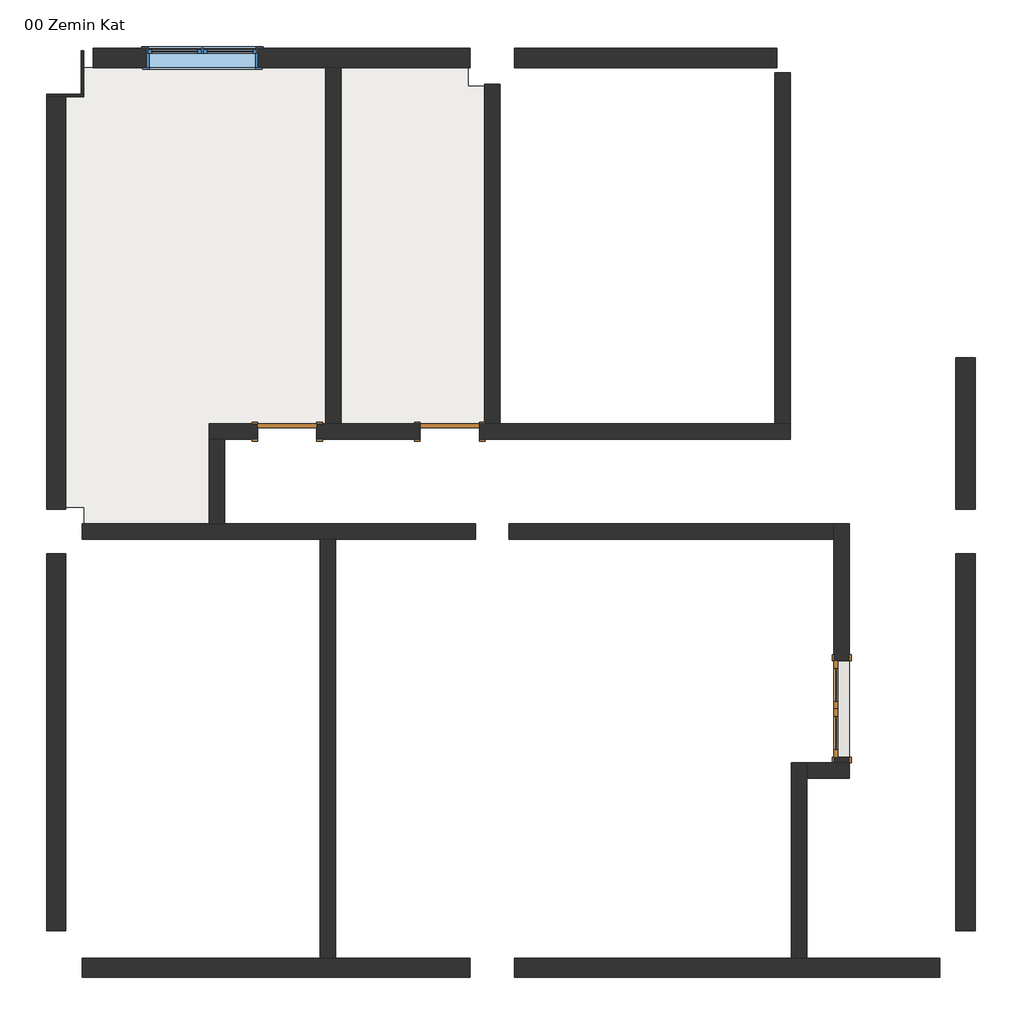
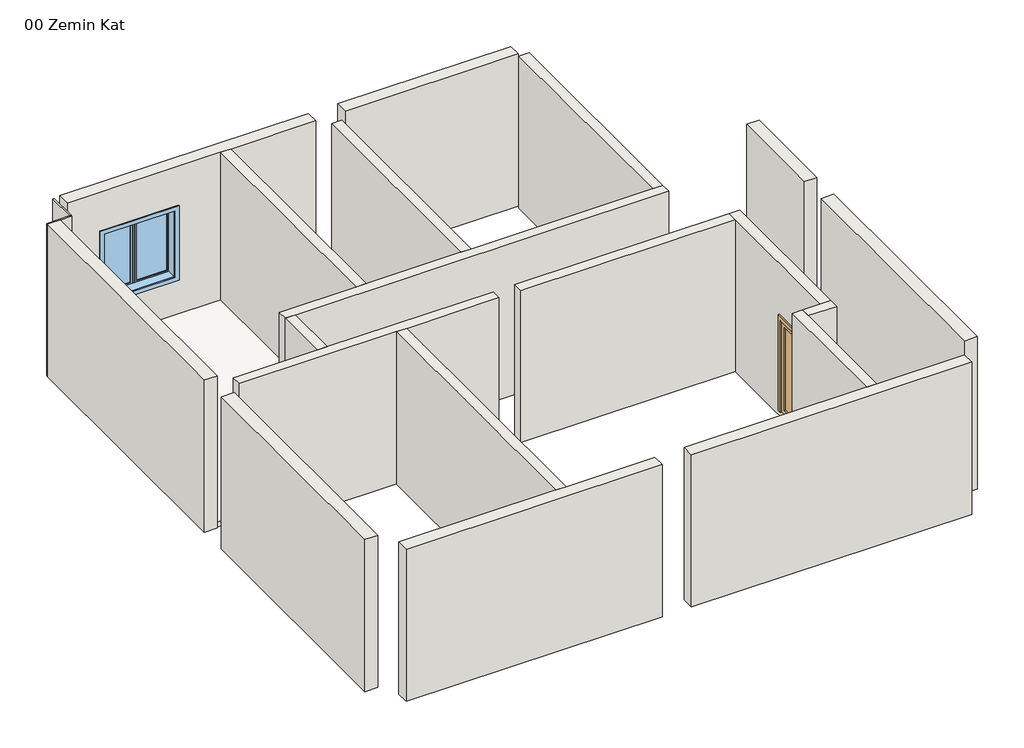
# One storey: 21 walls, 3 doors, 2 slabs, 1 window.
"""IFC4 building model written with IfcOpenShell, lengths in millimetres."""

import ifcopenshell
import ifcopenshell.guid

model = None  # the IFC model being written
_history = None  # IfcOwnerHistory: only IFC2X3 demands one
_inside = {}  # id of a spatial element -> (the spatial element, [elements in it])
_under = {}  # id of a project, library or spatial element -> (it, [spatial elements below it])
_declared = {}  # id of a project -> (the project, [libraries it declares])
_typed = {}  # id of a type object -> (the type object, [elements of that type])
_made_of = {}  # id of a material, layer set ... -> (it, [elements and type objects made of it])


def new_model(schema):
    """Start an empty IFC model of exactly this schema.

    Asked for "IFC4X3", IfcOpenShell would pick the latest addendum, in which some entities
    have other attributes; the version numbers below select the first issue.
    IFC2X3 requires an IfcOwnerHistory on every rooted entity: one is made here for all.
    """
    global model, _history
    if schema == "IFC4X3":
        model = ifcopenshell.file(schema_version=(4, 3, 0, 0))
    else:
        model = ifcopenshell.file(schema=schema)
    _inside.clear()
    _under.clear()
    _declared.clear()
    _typed.clear()
    _made_of.clear()
    _history = None
    if model.schema == "IFC2X3":
        org = make("IfcOrganization", Name="unknown")
        user = make(
            "IfcPersonAndOrganization",
            ThePerson=make("IfcPerson", FamilyName="unknown"),
            TheOrganization=org,
        )
        app = make(
            "IfcApplication",
            ApplicationDeveloper=org,
            Version="unknown",
            ApplicationFullName="unknown",
            ApplicationIdentifier="unknown",
        )
        _history = make(
            "IfcOwnerHistory",
            OwningUser=user,
            OwningApplication=app,
            ChangeAction="ADDED",
            CreationDate=0,
        )
    return model


def make(cls, **values):
    """One entity of the class cls with the attributes given. An attribute that is None is left unset."""
    return model.create_entity(
        cls, **{name: value for name, value in values.items() if value is not None}
    )


def rooted(cls, **values):
    """An entity with a GlobalId (a new one), such as an element, a storey or a relation."""
    return make(cls, GlobalId=ifcopenshell.guid.new(), OwnerHistory=_history, **values)


def si_unit(unit_type, name, prefix=None):
    """IfcSIUnit, for example si_unit("LENGTHUNIT", "METRE", prefix="MILLI")."""
    return make("IfcSIUnit", UnitType=unit_type, Prefix=prefix, Name=name)


def assignment(units):
    """IfcUnitAssignment: the units of a project."""
    return None if units is None else make("IfcUnitAssignment", Units=units)


def point(xyz):
    """IfcCartesianPoint."""
    return None if xyz is None else make("IfcCartesianPoint", Coordinates=xyz)


def direction(xyz):
    """IfcDirection."""
    return None if xyz is None else make("IfcDirection", DirectionRatios=xyz)


def frame(location, z_axis=None, x_axis=None):
    """IfcAxis2Placement3D, a coordinate frame: its origin and axes. An axis left out is left unset."""
    return make(
        "IfcAxis2Placement3D",
        Location=point(location),
        Axis=direction(z_axis),
        RefDirection=direction(x_axis),
    )


def origin():
    """The frame at (0, 0, 0) with its axes left unset."""
    return frame((0.0, 0.0, 0.0))


def origin_with_axes():
    """The frame at (0, 0, 0) with the z axis (0, 0, 1) and the x axis (1, 0, 0) written out."""
    return frame((0.0, 0.0, 0.0), z_axis=(0.0, 0.0, 1.0), x_axis=(1.0, 0.0, 0.0))


def place(relative_to, where):
    """IfcLocalPlacement: puts the frame where relative to a parent placement (None: the world)."""
    return make(
        "IfcLocalPlacement", PlacementRelTo=relative_to, RelativePlacement=where
    )


def context(
    kind, dimensions, precision=None, world=None, true_north=None, identifier=None
):
    """IfcGeometricRepresentationContext, for example the 3D "Model" context."""
    return make(
        "IfcGeometricRepresentationContext",
        ContextIdentifier=identifier,
        ContextType=kind,
        CoordinateSpaceDimension=dimensions,
        Precision=precision,
        WorldCoordinateSystem=world,
        TrueNorth=true_north,
    )


def project(units=None, contexts=None):
    """IfcProject with its units and contexts."""
    return rooted(
        "IfcProject",
        Name="project",
        RepresentationContexts=contexts,
        UnitsInContext=assignment(units),
    )


def spatial(cls, under=None, at=None, **own):
    """A site, building, storey or space (cls), placed at a placement, below another one or the project."""
    s = rooted(cls, ObjectPlacement=at, **own)
    if under is not None:
        _under.setdefault(under.id(), (under, []))[1].append(s)
    return s


def polyline(points):
    """IfcPolyline through the points."""
    return make("IfcPolyline", Points=[point(p) for p in points])


def outline(outer, holes=None, kind="AREA"):
    """IfcArbitraryClosedProfileDef: a profile drawn as a closed curve; with holes, ...WithVoids."""
    if holes is None:
        return make("IfcArbitraryClosedProfileDef", ProfileType=kind, OuterCurve=outer)
    return make(
        "IfcArbitraryProfileDefWithVoids",
        ProfileType=kind,
        OuterCurve=outer,
        InnerCurves=holes,
    )


def extrude(swept, where, along, depth):
    """IfcExtrudedAreaSolid: the profile swept, set in the frame where, extruded along a direction by depth."""
    return make(
        "IfcExtrudedAreaSolid",
        SweptArea=swept,
        Position=where,
        ExtrudedDirection=direction(along),
        Depth=depth,
    )


def faces_of(points, faces, orient=None, outer=None):
    """IfcFace entities. A face is a list of loops; a loop is a list of indices into points, from 0.

    orient and outer hold one flag for each loop. By default every Orientation is true, the
    first loop of a face is its IfcFaceOuterBound and the others are IfcFaceBound.
    """
    made = []
    for i, loops in enumerate(faces):
        bounds = []
        for j, loop in enumerate(loops):
            is_outer = j == 0 if outer is None else outer[i][j]
            bounds.append(
                make(
                    "IfcFaceOuterBound" if is_outer else "IfcFaceBound",
                    Bound=make("IfcPolyLoop", Polygon=[points[k] for k in loop]),
                    Orientation=True if orient is None else orient[i][j],
                )
            )
        made.append(make("IfcFace", Bounds=bounds))
    return made


def faceted_brep(points, faces, orient=None, outer=None, voids=None):
    """IfcFacetedBrep: a solid bounded by flat faces; with voids (closed shells), ...WithVoids."""
    shared = [point(p) for p in points]
    hull = make("IfcClosedShell", CfsFaces=faces_of(shared, faces, orient, outer))
    if voids is None:
        return make("IfcFacetedBrep", Outer=hull)
    return make(
        "IfcFacetedBrepWithVoids",
        Outer=hull,
        Voids=[
            make(cls, CfsFaces=faces_of(shared, fs, o, b)) for cls, fs, o, b in voids
        ],
    )


def shape(context_of_items, identifier, shape_type, items):
    """IfcShapeRepresentation: the items that make up one representation, for example the "Body"."""
    return make(
        "IfcShapeRepresentation",
        ContextOfItems=context_of_items,
        RepresentationIdentifier=identifier,
        RepresentationType=shape_type,
        Items=items,
    )


def source(mapping_origin, context_of_items, identifier, shape_type, items):
    """IfcRepresentationMap: a shape defined once, which mapped items show again and again."""
    return make(
        "IfcRepresentationMap",
        MappingOrigin=mapping_origin,
        MappedRepresentation=shape(context_of_items, identifier, shape_type, items),
    )


def transform(
    local_origin,
    x_axis=None,
    y_axis=None,
    z_axis=None,
    scale=None,
    scale2=None,
    scale3=None,
    uniform=True,
):
    """IfcCartesianTransformationOperator3D, or its non-uniform kind. x_axis, y_axis, z_axis: its Axis1, 2, 3."""
    if uniform:
        return make(
            "IfcCartesianTransformationOperator3D",
            Axis1=direction(x_axis),
            Axis2=direction(y_axis),
            LocalOrigin=point(local_origin),
            Scale=scale,
            Axis3=direction(z_axis),
        )
    return make(
        "IfcCartesianTransformationOperator3DnonUniform",
        Axis1=direction(x_axis),
        Axis2=direction(y_axis),
        LocalOrigin=point(local_origin),
        Scale=scale,
        Axis3=direction(z_axis),
        Scale2=scale2,
        Scale3=scale3,
    )


def mapped(mapping_source, mapping_target):
    """IfcMappedItem: shows the shape of a source again, moved by a transform."""
    return make(
        "IfcMappedItem", MappingSource=mapping_source, MappingTarget=mapping_target
    )


def made_of(thing, what):
    """Note that an element or type object is made of a material, layer set ...; save() writes the relation."""
    if what is not None:
        _made_of.setdefault(what.id(), (what, []))[1].append(thing)
    return thing


def element(
    cls,
    number,
    at=None,
    inside=None,
    cuts=None,
    type_object=None,
    material=None,
    context=None,
    identifier="Body",
    shape_type=None,
    held_by="IfcProductDefinitionShape",
    body=None,
    shapes=None,
    **own,
):
    """One element of the class cls, such as IfcWall. Its Tag is "e" and its number.

    at: its placement. inside: the storey or other place that contains it. cuts: it is an
    opening in that element (IfcRelVoidsElement). A single representation is given by context,
    identifier, shape_type and body (its items); several are given by shapes. held_by: the class
    of the entity that holds the representations. save() writes the other relations.
    """
    e = rooted(cls, Tag="e%d" % number, ObjectPlacement=at, **own)
    if body is not None:
        shapes = [shape(context, identifier, shape_type, body)]
    if shapes is not None:
        e.Representation = make(held_by, Representations=shapes)
    if inside is not None:
        _inside.setdefault(inside.id(), (inside, []))[1].append(e)
    if cuts is not None:
        rooted(
            "IfcRelVoidsElement", RelatingBuildingElement=cuts, RelatedOpeningElement=e
        )
    if type_object is not None:
        _typed.setdefault(type_object.id(), (type_object, []))[1].append(e)
    return made_of(e, material)


def aggregate(whole, parts):
    """IfcRelAggregates: a whole, such as a stair, and the parts it consists of."""
    return rooted("IfcRelAggregates", RelatingObject=whole, RelatedObjects=parts)


def save(model, path):
    """Write the relations noted so far, then the file.

    IfcRelAggregates (storeys below a building ...), IfcRelContainedInSpatialStructure (elements
    in a storey), IfcRelDefinesByType, IfcRelAssociatesMaterial and IfcRelDeclares: one each for
    every whole, place, type object, material and project.
    """
    for whole, parts in _under.values():
        aggregate(whole, parts)
    for where, things in _inside.values():
        rooted(
            "IfcRelContainedInSpatialStructure",
            RelatedElements=things,
            RelatingStructure=where,
        )
    for kind, things in _typed.values():
        rooted("IfcRelDefinesByType", RelatedObjects=things, RelatingType=kind)
    for what, things in _made_of.values():
        rooted("IfcRelAssociatesMaterial", RelatedObjects=things, RelatingMaterial=what)
    for by, libraries in _declared.values():
        rooted("IfcRelDeclares", RelatingContext=by, RelatedDefinitions=libraries)
    model.write(path)


def m_door_double_glass_87eabaac(model_context):
    return source(origin(), model_context, "Body", "SweptSolid", [
        extrude(outline(polyline([(2000.0, -650.0), (0.0, -650.0), (0.0, 0.0), (2000.0, 0.0), (2000.0, -650.0)]), holes=[polyline([(1900.0, -550.0), (1900.0, -100.0), (100.0, -100.0), (100.0, -550.0), (1900.0, -550.0)])]), frame((0.0, 57.38125, 0.0), z_axis=(0.0, 1.0, 0.0), x_axis=(0.0, 0.0, 1.0)), (0.0, 0.0, 1.0), 50.0),
        extrude(outline(polyline([(2000.0, 650.0), (2000.0, 0.0), (0.0, 0.0), (0.0, 650.0), (2000.0, 650.0)]), holes=[polyline([(1900.0, 550.0), (100.0, 550.0), (100.0, 100.0), (1900.0, 100.0), (1900.0, 550.0)])]), frame((0.0, 57.38125, 0.0), z_axis=(0.0, 1.0, 0.0), x_axis=(0.0, 0.0, 1.0)), (0.0, 0.0, 1.0), 50.0),
        extrude(outline(polyline([(100.0, 85.55625), (550.0, 85.55625), (550.0, 79.20625), (100.0, 79.20625), (100.0, 85.55625)])), frame((0.0, 0.0, 100.0), z_axis=(0.0, 0.0, 1.0), x_axis=(1.0, 0.0, 0.0)), (0.0, 0.0, 1.0), 1800.0),
        extrude(outline(polyline([(-550.0, 85.55625), (-100.0, 85.55625), (-100.0, 79.20625), (-550.0, 79.20625), (-550.0, 85.55625)])), frame((0.0, 0.0, 100.0), z_axis=(0.0, 0.0, 1.0), x_axis=(1.0, 0.0, 0.0)), (0.0, 0.0, 1.0), 1800.0),
        extrude(outline(polyline([(0.0, 730.0), (2080.0, 730.0), (2080.0, -730.0), (0.0, -730.0), (0.0, -650.0), (2000.0, -650.0), (2000.0, 650.0), (0.0, 650.0), (0.0, 730.0)])), frame((0.0, 107.38125, 0.0), z_axis=(0.0, 1.0, 0.0), x_axis=(0.0, 0.0, 1.0)), (0.0, 0.0, 1.0), 25.0),
        extrude(outline(polyline([(0.0, 730.0), (2080.0, 730.0), (2080.0, -730.0), (0.0, -730.0), (0.0, -650.0), (2000.0, -650.0), (2000.0, 650.0), (0.0, 650.0), (0.0, 730.0)])), frame((0.0, -127.61875, 0.0), z_axis=(0.0, 1.0, 0.0), x_axis=(0.0, 0.0, 1.0)), (0.0, 0.0, 1.0), 25.0),
    ])


def m_single_flush_43d1bd44(model_context):
    return source(origin(), model_context, "Body", "SweptSolid", [
        extrude(outline(polyline([(2176.0, -476.0), (0.0, -476.0), (0.0, -400.0), (2100.0, -400.0), (2100.0, 400.0), (0.0, 400.0), (0.0, 476.0), (2176.0, 476.0), (2176.0, -476.0)])), frame((0.0, 105.0, 0.0), z_axis=(0.0, 1.0, 0.0), x_axis=(0.0, 0.0, 1.0)), (0.0, 0.0, 1.0), 25.0),
        extrude(outline(polyline([(2176.0, 476.0), (2176.0, -476.0), (0.0, -476.0), (0.0, -400.0), (2100.0, -400.0), (2100.0, 400.0), (0.0, 400.0), (0.0, 476.0), (2176.0, 476.0)])), frame((0.0, -130.0, 0.0), z_axis=(0.0, 1.0, 0.0), x_axis=(0.0, 0.0, 1.0)), (0.0, 0.0, 1.0), 25.0),
        extrude(outline(polyline([(400.0, 54.0), (-400.0, 54.0), (-400.0, 105.0), (400.0, 105.0), (400.0, 54.0)])), origin_with_axes(), (0.0, 0.0, 1.0), 2100.0),
    ])


def m_casement_dbl_with_trim_011da180(model_context):
    return source(origin(), model_context, "Body", "SweptSolid", [
        extrude(outline(polyline([(63.5, 114.175), (686.5, 114.175), (686.5, 101.475), (63.5, 101.475), (63.5, 114.175)])), frame((0.0, 0.0, 978.5), z_axis=(0.0, 0.0, 1.0), x_axis=(1.0, 0.0, 0.0)), (0.0, 0.0, 1.0), 1373.0),
        extrude(outline(polyline([(2395.95, 19.05), (934.05, 19.05), (934.05, 730.95), (2395.95, 730.95), (2395.95, 19.05)]), holes=[polyline([(2351.5, 63.5), (2351.5, 686.5), (978.5, 686.5), (978.5, 63.5), (2351.5, 63.5)])]), frame((0.0, 85.6, 0.0), z_axis=(0.0, 1.0, 0.0), x_axis=(0.0, 0.0, 1.0)), (0.0, 0.0, 1.0), 44.45),
        extrude(outline(polyline([(-819.95, 174.75), (819.95, 174.75), (819.95, 149.05), (-819.95, 149.05), (-819.95, 174.75)])), frame((0.0, 0.0, 915.0), z_axis=(0.0, 0.0, 1.0), x_axis=(1.0, 0.0, 0.0)), (0.0, 0.0, 1.0), 19.05),
        extrude(outline(polyline([(2395.95, -730.95), (2395.95, 730.95), (934.05, 730.95), (934.05, 819.95), (2484.95, 819.95), (2484.95, -819.95), (934.05, -819.95), (934.05, -730.95), (2395.95, -730.95)])), frame((0.0, 149.05, 0.0), z_axis=(0.0, 1.0, 0.0), x_axis=(0.0, 0.0, 1.0)), (0.0, 0.0, 1.0), 13.0),
        extrude(outline(polyline([(2472.25, 807.25), (2472.25, -807.25), (857.75, -807.25), (857.75, 807.25), (2472.25, 807.25)]), holes=[polyline([(2383.25, 718.25), (946.75, 718.25), (946.75, -718.25), (2383.25, -718.25), (2383.25, 718.25)])]), frame((0.0, -129.95, 0.0), z_axis=(0.0, 1.0, 0.0), x_axis=(0.0, 0.0, 1.0)), (0.0, 0.0, 1.0), 19.0),
        extrude(outline(polyline([(-63.5, 101.475), (-686.5, 101.475), (-686.5, 114.175), (-63.5, 114.175), (-63.5, 101.475)])), frame((0.0, 0.0, 978.5), z_axis=(0.0, 0.0, 1.0), x_axis=(1.0, 0.0, 0.0)), (0.0, 0.0, 1.0), 1373.0),
        extrude(outline(polyline([(2395.95, -730.95), (934.05, -730.95), (934.05, -19.05), (2395.95, -19.05), (2395.95, -730.95)]), holes=[polyline([(2351.5, -686.5), (2351.5, -63.5), (978.5, -63.5), (978.5, -686.5), (2351.5, -686.5)])]), frame((0.0, 85.6, 0.0), z_axis=(0.0, 1.0, 0.0), x_axis=(0.0, 0.0, 1.0)), (0.0, 0.0, 1.0), 44.45),
        extrude(outline(polyline([(2415.0, -750.0), (915.0, -750.0), (915.0, 750.0), (2415.0, 750.0), (2415.0, -750.0)]), holes=[polyline([(2383.25, -718.25), (2383.25, 718.25), (946.75, 718.25), (946.75, -718.25), (2383.25, -718.25)])]), frame((0.0, -110.95, 0.0), z_axis=(0.0, 1.0, 0.0), x_axis=(0.0, 0.0, 1.0)), (0.0, 0.0, 1.0), 196.55),
        extrude(outline(polyline([(2415.0, 750.0), (2415.0, -750.0), (915.0, -750.0), (915.0, 750.0), (2415.0, 750.0)]), holes=[polyline([(2395.95, 730.95), (934.05, 730.95), (934.05, -730.95), (2395.95, -730.95), (2395.95, 730.95)])]), frame((0.0, 85.6, 0.0), z_axis=(0.0, 1.0, 0.0), x_axis=(0.0, 0.0, 1.0)), (0.0, 0.0, 1.0), 63.45),
        extrude(outline(polyline([(19.05, 85.6), (-19.05, 85.6), (-19.05, 149.1), (19.05, 149.1), (19.05, 85.6)])), frame((0.0, 0.0, 934.05), z_axis=(0.0, 0.0, 1.0), x_axis=(1.0, 0.0, 0.0)), (0.0, 0.0, 1.0), 1461.9),
    ])


model = new_model("IFC4")

# Units and contexts
model_context = context("Model", 3, world=origin())
ifc_project = project(units=[si_unit("LENGTHUNIT", "METRE", prefix="MILLI")], contexts=[model_context])

# Site, building, storey
site = spatial("IfcSite", under=ifc_project)
building = spatial("IfcBuilding", under=site)
storey = spatial("IfcBuildingStorey", under=building, Name="00 Zemin Kat", Elevation=93780.0)

# Doors
placement = place(None, origin())
m_door_double_glass_shape = m_door_double_glass_87eabaac(model_context)
element("IfcDoor", 1, ObjectType="M_Door-Double-Glass : 130x210cm Kapı", at=placement, inside=storey, context=model_context, shape_type="MappedRepresentation", body=[
    mapped(m_door_double_glass_shape, transform((-4449.1672628, -121.7095574, 93900.0), x_axis=(0.0, 1.0, 0.0), y_axis=(-1.0, 0.0, 0.0), z_axis=(0.0, 0.0, 1.0))),
])
m_single_flush_shape = m_single_flush_43d1bd44(model_context)
element("IfcDoor", 2, ObjectType="M_Single-Flush : 90x210cm Kapı", at=placement, inside=storey, context=model_context, shape_type="MappedRepresentation", body=[
    mapped(m_single_flush_shape, transform((-11954.0485128, 3626.2599093, 93780.0), x_axis=(1.0, 0.0, 0.0), y_axis=(0.0, 1.0, 0.0), z_axis=(0.0, 0.0, 1.0))),
])
element("IfcDoor", 3, ObjectType="M_Single-Flush : 90x210cm Kapı", at=placement, inside=storey, context=model_context, shape_type="MappedRepresentation", body=[
    mapped(m_single_flush_shape, transform((-9754.0485128, 3626.2599093, 93780.0), x_axis=(1.0, 0.0, 0.0), y_axis=(0.0, 1.0, 0.0), z_axis=(0.0, 0.0, 1.0))),
])

# Slabs
element("IfcSlab", 4, ObjectType="10cm Parke", at=placement, inside=storey, context=model_context, shape_type="SweptSolid", body=[
    extrude(outline(polyline([(-14699.0485128, 8548.2904426), (-11434.0485128, 8548.2904426), (-11434.0485128, 3731.2599093), (-13009.0485128, 3731.2599093), (-13009.0485128, 2383.2904426), (-14699.0485128, 2383.2904426), (-14699.0485128, 2608.2904426), (-14949.0485128, 2608.2904426), (-14949.0485128, 8148.2904426), (-14699.0485128, 8148.2904426), (-14699.0485128, 8548.2904426)])), frame((0.0, 0.0, 93780.0), z_axis=(0.0, 0.0, 1.0), x_axis=(1.0, 0.0, 0.0)), (0.0, 0.0, 1.0), 100.0),
])
element("IfcSlab", 5, ObjectType="10cm Seramik", at=placement, inside=storey, context=model_context, shape_type="SweptSolid", body=[
    extrude(outline(polyline([(-9509.0485128, 8548.2904426), (-9509.0485128, 8298.2904426), (-9284.0485128, 8298.2904426), (-9284.0485128, 3731.2599093), (-11224.0485128, 3731.2599093), (-11224.0485128, 8548.2904426), (-9509.0485128, 8548.2904426)])), frame((0.0, 0.0, 93780.0), z_axis=(0.0, 0.0, 1.0), x_axis=(1.0, 0.0, 0.0)), (0.0, 0.0, 1.0), 100.0),
])

# Walls
element("IfcWall", 6, ObjectType="Dış Duvar_26cm", at=placement, inside=storey, context=model_context, shape_type="Brep", body=[
    faceted_brep([(-14579.0485128, 8548.2904426, 93780.0), (-11434.0485128, 8548.2904426, 93780.0), (-11224.0485128, 8548.2904426, 93780.0), (-9479.0485128, 8548.2904426, 93780.0), (-9479.0485128, 8548.2904426, 97080.0), (-11224.0485128, 8548.2904426, 97080.0), (-11434.0485128, 8548.2904426, 97080.0), (-14579.0485128, 8548.2904426, 97080.0), (-12351.5235128, 8548.2904426, 96180.0), (-12351.5235128, 8548.2904426, 94680.0), (-13851.5235128, 8548.2904426, 94680.0), (-13851.5235128, 8548.2904426, 96180.0), (-14579.0485128, 8808.2904426, 93780.0), (-14579.0485128, 8808.2904426, 97080.0), (-9479.0485128, 8808.2904426, 97080.0), (-9479.0485128, 8808.2904426, 93780.0), (-12351.5235128, 8808.2904426, 96180.0), (-13851.5235128, 8808.2904426, 96180.0), (-13851.5235128, 8808.2904426, 94680.0), (-12351.5235128, 8808.2904426, 94680.0)], [[[0, 1, 2, 3, 4, 5, 6, 7], [8, 9, 10, 11]], [[12, 13, 14, 15], [16, 17, 18, 19]], [[3, 2, 1, 0, 12, 15]], [[4, 3, 15, 14]], [[7, 6, 5, 4, 14, 13]], [[0, 7, 13, 12]], [[9, 8, 16, 19]], [[10, 9, 19, 18]], [[11, 10, 18, 17]], [[8, 11, 17, 16]]]),
])
element("IfcWall", 7, ObjectType="Dış Duvar_26cm", at=placement, inside=storey, context=model_context, shape_type="SweptSolid", body=[
    extrude(outline(polyline([(-5329.0485128, 8548.2904426), (-8879.0485128, 8548.2904426), (-8879.0485128, 8808.2904426), (-5329.0485128, 8808.2904426), (-5329.0485128, 8548.2904426)])), frame((0.0, 0.0, 93780.0), z_axis=(0.0, 0.0, 1.0), x_axis=(1.0, 0.0, 0.0)), (0.0, 0.0, 1.0), 3300.0),
])
element("IfcWall", 8, ObjectType="Dış Duvar_26cm", at=placement, inside=storey, context=model_context, shape_type="SweptSolid", body=[
    extrude(outline(polyline([(-2909.0485128, 2578.2904426), (-2909.0485128, 4628.2904426), (-2649.0485128, 4628.2904426), (-2649.0485128, 2578.2904426), (-2909.0485128, 2578.2904426)])), frame((0.0, 0.0, 93780.0), z_axis=(0.0, 0.0, 1.0), x_axis=(1.0, 0.0, 0.0)), (0.0, 0.0, 1.0), 3300.0),
])
element("IfcWall", 9, ObjectType="Dış Duvar_26cm", at=placement, inside=storey, context=model_context, shape_type="SweptSolid", body=[
    extrude(outline(polyline([(-2909.0485128, -3121.7095574), (-2909.0485128, 1978.2904426), (-2649.0485128, 1978.2904426), (-2649.0485128, -3121.7095574), (-2909.0485128, -3121.7095574)])), frame((0.0, 0.0, 93780.0), z_axis=(0.0, 0.0, 1.0), x_axis=(1.0, 0.0, 0.0)), (0.0, 0.0, 1.0), 3300.0),
])
element("IfcWall", 10, ObjectType="Dış Duvar_26cm", at=placement, inside=storey, context=model_context, shape_type="Brep", body=[
    faceted_brep([(-3129.0485128, -3491.7095574, 93780.0), (-4926.5485128, -3491.7095574, 93780.0), (-5136.5485128, -3491.7095574, 93780.0), (-8879.0485128, -3491.7095574, 93780.0), (-8879.0485128, -3491.7095574, 97080.0), (-5136.5485128, -3491.7095574, 97080.0), (-4926.5485128, -3491.7095574, 97080.0), (-3129.0485128, -3491.7095574, 97080.0), (-3129.0485128, -3751.7095574, 93780.0), (-3129.0485128, -3751.7095574, 97080.0), (-8879.0485128, -3751.7095574, 97080.0), (-8879.0485128, -3751.7095574, 93780.0)], [[[0, 1, 2, 3, 4, 5, 6, 7]], [[8, 9, 10, 11]], [[3, 2, 1, 0, 8, 11]], [[4, 3, 11, 10]], [[7, 6, 5, 4, 10, 9]], [[0, 7, 9, 8]]]),
])
element("IfcWall", 11, ObjectType="Dış Duvar_26cm", at=placement, inside=storey, context=model_context, shape_type="Brep", body=[
    faceted_brep([(-9479.0485128, -3491.7095574, 93780.0), (-11299.0485128, -3491.7095574, 93780.0), (-11509.0485128, -3491.7095574, 93780.0), (-14729.0485128, -3491.7095574, 93780.0), (-14729.0485128, -3491.7095574, 97080.0), (-11509.0485128, -3491.7095574, 97080.0), (-11299.0485128, -3491.7095574, 97080.0), (-9479.0485128, -3491.7095574, 97080.0), (-9479.0485128, -3751.7095574, 93780.0), (-9479.0485128, -3751.7095574, 97080.0), (-14729.0485128, -3751.7095574, 97080.0), (-14729.0485128, -3751.7095574, 93780.0)], [[[0, 1, 2, 3, 4, 5, 6, 7]], [[8, 9, 10, 11]], [[3, 2, 1, 0, 8, 11]], [[4, 3, 11, 10]], [[7, 6, 5, 4, 10, 9]], [[0, 7, 9, 8]]]),
])
element("IfcWall", 12, ObjectType="Dış Duvar_26cm", at=placement, inside=storey, context=model_context, shape_type="SweptSolid", body=[
    extrude(outline(polyline([(-14949.0485128, 1978.2904426), (-14949.0485128, -3121.7095574), (-15209.0485128, -3121.7095574), (-15209.0485128, 1978.2904426), (-14949.0485128, 1978.2904426)])), frame((0.0, 0.0, 93780.0), z_axis=(0.0, 0.0, 1.0), x_axis=(1.0, 0.0, 0.0)), (0.0, 0.0, 1.0), 3300.0),
])
element("IfcWall", 13, ObjectType="Dış Duvar_26cm", at=placement, inside=storey, context=model_context, shape_type="SweptSolid", body=[
    extrude(outline(polyline([(-14949.0485128, 8155.7904426), (-14949.0485128, 2578.2904426), (-15209.0485128, 2578.2904426), (-15209.0485128, 8155.7904426), (-14949.0485128, 8155.7904426)])), frame((0.0, 0.0, 93780.0), z_axis=(0.0, 0.0, 1.0), x_axis=(1.0, 0.0, 0.0)), (0.0, 0.0, 1.0), 3300.0),
])
element("IfcWall", 14, ObjectType="İç Duvar_21cm", at=placement, inside=storey, context=model_context, shape_type="SweptSolid", body=[
    extrude(outline(polyline([(-11434.0485128, 3731.2599093), (-11434.0485128, 8548.2904426), (-11224.0485128, 8548.2904426), (-11224.0485128, 3731.2599093), (-11434.0485128, 3731.2599093)])), frame((0.0, 0.0, 93780.0), z_axis=(0.0, 0.0, 1.0), x_axis=(1.0, 0.0, 0.0)), (0.0, 0.0, 1.0), 3300.0),
])
element("IfcWall", 15, ObjectType="İç Duvar_21cm", at=placement, inside=storey, context=model_context, shape_type="Brep", body=[
    faceted_brep([(-9354.0485128, 3521.2599093, 95880.0), (-9354.0485128, 3521.2599093, 93780.0), (-5144.0485128, 3521.2599093, 93780.0), (-5144.0485128, 3521.2599093, 97080.0), (-12799.0485128, 3521.2599093, 97080.0), (-13009.0485128, 3521.2599093, 97080.0), (-13009.0485128, 3521.2599093, 93780.0), (-12799.0485128, 3521.2599093, 93780.0), (-12354.0485128, 3521.2599093, 93780.0), (-12354.0485128, 3521.2599093, 95880.0), (-11554.0485128, 3521.2599093, 95880.0), (-11554.0485128, 3521.2599093, 93780.0), (-10154.0485128, 3521.2599093, 93780.0), (-10154.0485128, 3521.2599093, 95880.0), (-5144.0485128, 3731.2599093, 93780.0), (-5354.0485128, 3731.2599093, 93780.0), (-9074.0485128, 3731.2599093, 93780.0), (-9284.0485128, 3731.2599093, 93780.0), (-9354.0485128, 3731.2599093, 93780.0), (-9354.0485128, 3731.2599093, 95880.0), (-10154.0485128, 3731.2599093, 95880.0), (-10154.0485128, 3731.2599093, 93780.0), (-11224.0485128, 3731.2599093, 93780.0), (-11434.0485128, 3731.2599093, 93780.0), (-11554.0485128, 3731.2599093, 93780.0), (-11554.0485128, 3731.2599093, 95880.0), (-12354.0485128, 3731.2599093, 95880.0), (-12354.0485128, 3731.2599093, 93780.0), (-13009.0485128, 3731.2599093, 93780.0), (-13009.0485128, 3731.2599093, 97080.0), (-11434.0485128, 3731.2599093, 97080.0), (-11224.0485128, 3731.2599093, 97080.0), (-9284.0485128, 3731.2599093, 97080.0), (-9074.0485128, 3731.2599093, 97080.0), (-5354.0485128, 3731.2599093, 97080.0), (-5144.0485128, 3731.2599093, 97080.0)], [[[0, 1, 2, 3, 4, 5, 6, 7, 8, 9, 10, 11, 12, 13]], [[14, 15, 16, 17, 18, 19, 20, 21, 22, 23, 24, 25, 26, 27, 28, 29, 30, 31, 32, 33, 34, 35]], [[8, 7, 6, 28, 27]], [[12, 11, 24, 23, 22, 21]], [[2, 1, 18, 17, 16, 15, 14]], [[5, 4, 3, 35, 34, 33, 32, 31, 30, 29]], [[3, 2, 14, 35]], [[6, 5, 29, 28]], [[25, 24, 11, 10]], [[26, 25, 10, 9]], [[27, 26, 9, 8]], [[19, 18, 1, 0]], [[20, 19, 0, 13]], [[21, 20, 13, 12]]]),
])
element("IfcWall", 16, ObjectType="İç Duvar_21cm", at=placement, inside=storey, context=model_context, shape_type="SweptSolid", body=[
    extrude(outline(polyline([(-5144.0485128, 8478.2904426), (-5144.0485128, 3731.2599093), (-5354.0485128, 3731.2599093), (-5354.0485128, 8478.2904426), (-5144.0485128, 8478.2904426)])), frame((0.0, 0.0, 93780.0), z_axis=(0.0, 0.0, 1.0), x_axis=(1.0, 0.0, 0.0)), (0.0, 0.0, 1.0), 3300.0),
])
element("IfcWall", 17, ObjectType="İç Duvar_21cm", at=placement, inside=storey, context=model_context, shape_type="SweptSolid", body=[
    extrude(outline(polyline([(-9284.0485128, 3731.2599093), (-9284.0485128, 8327.5055023), (-9074.0485128, 8327.5055023), (-9074.0485128, 3731.2599093), (-9284.0485128, 3731.2599093)])), frame((0.0, 0.0, 93780.0), z_axis=(0.0, 0.0, 1.0), x_axis=(1.0, 0.0, 0.0)), (0.0, 0.0, 1.0), 3300.0),
])
element("IfcWall", 18, ObjectType="İç Duvar_21cm", at=placement, inside=storey, context=model_context, shape_type="SweptSolid", body=[
    extrude(outline(polyline([(-13009.0485128, 2383.2904426), (-13009.0485128, 3521.2599093), (-12799.0485128, 3521.2599093), (-12799.0485128, 2383.2904426), (-13009.0485128, 2383.2904426)])), frame((0.0, 0.0, 93780.0), z_axis=(0.0, 0.0, 1.0), x_axis=(1.0, 0.0, 0.0)), (0.0, 0.0, 1.0), 3300.0),
])
element("IfcWall", 19, ObjectType="İç Duvar_21cm", at=placement, inside=storey, context=model_context, shape_type="Brep", body=[
    faceted_brep([(-9404.0485128, 2383.2904426, 93780.0), (-12799.0485128, 2383.2904426, 93780.0), (-13009.0485128, 2383.2904426, 93780.0), (-14729.0485128, 2383.2904426, 93780.0), (-14729.0485128, 2383.2904426, 97080.0), (-13009.0485128, 2383.2904426, 97080.0), (-12799.0485128, 2383.2904426, 97080.0), (-9404.0485128, 2383.2904426, 97080.0), (-9404.0485128, 2173.2904426, 93780.0), (-9404.0485128, 2173.2904426, 97080.0), (-11299.0485128, 2173.2904426, 97080.0), (-11509.0485128, 2173.2904426, 97080.0), (-14729.0485128, 2173.2904426, 97080.0), (-14729.0485128, 2173.2904426, 93780.0), (-11509.0485128, 2173.2904426, 93780.0), (-11299.0485128, 2173.2904426, 93780.0)], [[[0, 1, 2, 3, 4, 5, 6, 7]], [[8, 9, 10, 11, 12, 13, 14, 15]], [[3, 2, 1, 0, 8, 15, 14, 13]], [[4, 3, 13, 12]], [[7, 6, 5, 4, 12, 11, 10, 9]], [[0, 7, 9, 8]]]),
])
element("IfcWall", 20, ObjectType="İç Duvar_21cm", at=placement, inside=storey, context=model_context, shape_type="SweptSolid", body=[
    extrude(outline(polyline([(-11509.0485128, -3491.7095574), (-11509.0485128, 2173.2904426), (-11299.0485128, 2173.2904426), (-11299.0485128, -3491.7095574), (-11509.0485128, -3491.7095574)])), frame((0.0, 0.0, 93780.0), z_axis=(0.0, 0.0, 1.0), x_axis=(1.0, 0.0, 0.0)), (0.0, 0.0, 1.0), 3300.0),
])
element("IfcWall", 21, ObjectType="İç Duvar_21cm", at=placement, inside=storey, context=model_context, shape_type="Brep", body=[
    faceted_brep([(-4926.5485128, -3491.7095574, 93780.0), (-4926.5485128, -1056.7095574, 93780.0), (-4926.5485128, -846.7095574, 93780.0), (-4926.5485128, -846.7095574, 97080.0), (-4926.5485128, -1056.7095574, 97080.0), (-4926.5485128, -3491.7095574, 97080.0), (-5136.5485128, -3491.7095574, 93780.0), (-5136.5485128, -3491.7095574, 97080.0), (-5136.5485128, -846.7095574, 97080.0), (-5136.5485128, -846.7095574, 93780.0)], [[[0, 1, 2, 3, 4, 5]], [[6, 7, 8, 9]], [[2, 1, 0, 6, 9]], [[5, 4, 3, 8, 7]], [[0, 5, 7, 6]], [[3, 2, 9, 8]]]),
])
element("IfcWall", 22, ObjectType="İç Duvar_21cm", at=placement, inside=storey, context=model_context, shape_type="Brep", body=[
    faceted_brep([(-4926.5485128, -1056.7095574, 93780.0), (-4346.5485128, -1056.7095574, 93780.0), (-4346.5485128, -1056.7095574, 97080.0), (-4926.5485128, -1056.7095574, 97080.0), (-4926.5485128, -846.7095574, 93780.0), (-4926.5485128, -846.7095574, 97080.0), (-4556.5485128, -846.7095574, 97080.0), (-4346.5485128, -846.7095574, 97080.0), (-4346.5485128, -846.7095574, 93780.0), (-4556.5485128, -846.7095574, 93780.0)], [[[0, 1, 2, 3]], [[4, 5, 6, 7, 8, 9]], [[1, 0, 4, 9, 8]], [[3, 2, 7, 6, 5]], [[0, 3, 5, 4]], [[2, 1, 8, 7]]]),
])
element("IfcWall", 23, ObjectType="İç Duvar_21cm", at=placement, inside=storey, context=model_context, shape_type="Brep", body=[
    faceted_brep([(-4346.5485128, -846.7095574, 93780.0), (-4346.5485128, 2383.2904426, 93780.0), (-4346.5485128, 2383.2904426, 97080.0), (-4346.5485128, -846.7095574, 97080.0), (-4346.5485128, 528.2904426, 93900.0), (-4346.5485128, -771.7095574, 93900.0), (-4346.5485128, -771.7095574, 95900.0), (-4346.5485128, 528.2904426, 95900.0), (-4556.5485128, 2383.2904426, 93780.0), (-4556.5485128, 2173.2904426, 93780.0), (-4556.5485128, -846.7095574, 93780.0), (-4556.5485128, -846.7095574, 97080.0), (-4556.5485128, 2173.2904426, 97080.0), (-4556.5485128, 2383.2904426, 97080.0), (-4556.5485128, -771.7095574, 93900.0), (-4556.5485128, 528.2904426, 93900.0), (-4556.5485128, 528.2904426, 95900.0), (-4556.5485128, -771.7095574, 95900.0)], [[[0, 1, 2, 3], [4, 5, 6, 7]], [[8, 9, 10, 11, 12, 13], [14, 15, 16, 17]], [[1, 0, 10, 9, 8]], [[3, 2, 13, 12, 11]], [[0, 3, 11, 10]], [[2, 1, 8, 13]], [[14, 5, 4, 15]], [[15, 4, 7, 16]], [[16, 7, 6, 17]], [[5, 14, 17, 6]]]),
])
element("IfcWall", 24, ObjectType="İç Duvar_21cm", at=placement, inside=storey, context=model_context, shape_type="SweptSolid", body=[
    extrude(outline(polyline([(-8954.0485128, 2383.2904426), (-4556.5485128, 2383.2904426), (-4556.5485128, 2173.2904426), (-8954.0485128, 2173.2904426), (-8954.0485128, 2383.2904426)])), frame((0.0, 0.0, 93780.0), z_axis=(0.0, 0.0, 1.0), x_axis=(1.0, 0.0, 0.0)), (0.0, 0.0, 1.0), 3300.0),
])
element("IfcWall", 25, ObjectType="Kolon Çevresi 3cm", at=placement, inside=storey, context=model_context, shape_type="Brep", body=[
    faceted_brep([(-15209.0485128, 8155.7904426, 93780.0), (-14949.0485128, 8155.7904426, 93780.0), (-14706.5485128, 8155.7904426, 93780.0), (-14706.5485128, 8155.7904426, 97080.0), (-14949.0485128, 8155.7904426, 97080.0), (-15209.0485128, 8155.7904426, 97080.0), (-15209.0485128, 8185.7904426, 93780.0), (-15209.0485128, 8185.7904426, 97080.0), (-14736.5485128, 8185.7904426, 97080.0), (-14706.5485128, 8185.7904426, 97080.0), (-14706.5485128, 8185.7904426, 93780.0), (-14736.5485128, 8185.7904426, 93780.0)], [[[0, 1, 2, 3, 4, 5]], [[6, 7, 8, 9, 10, 11]], [[2, 1, 0, 6, 11, 10]], [[5, 4, 3, 9, 8, 7]], [[0, 5, 7, 6]], [[3, 2, 10, 9]]]),
])
element("IfcWall", 26, ObjectType="Kolon Çevresi 3cm", at=placement, inside=storey, context=model_context, shape_type="SweptSolid", body=[
    extrude(outline(polyline([(-14706.5485128, 8778.2904426), (-14706.5485128, 8185.7904426), (-14736.5485128, 8185.7904426), (-14736.5485128, 8778.2904426), (-14706.5485128, 8778.2904426)])), frame((0.0, 0.0, 93780.0), z_axis=(0.0, 0.0, 1.0), x_axis=(1.0, 0.0, 0.0)), (0.0, 0.0, 1.0), 3300.0),
])

# Window
m_casement_dbl_with_trim_shape = m_casement_dbl_with_trim_011da180(model_context)
element("IfcWindow", 27, ObjectType="M_Casement Dbl with Trim : 150x150cm Pencere", at=placement, inside=storey, context=model_context, shape_type="MappedRepresentation", body=[
    mapped(m_casement_dbl_with_trim_shape, transform((-13101.5235128, 8659.2404426, 93765.0), x_axis=(1.0, 0.0, 0.0), y_axis=(0.0, 1.0, 0.0), z_axis=(0.0, 0.0, 1.0))),
])

save(model, "model.ifc")

# Revit data of these elements
# Project information
#   Project Issue Date = "Issue Date"
#   Project Status = "Project Status"
#   Client Name = "Owner"
#   Project Address = "Enter address here"
#   Project Name = "Project Name"
#   Project Number = "0001"
# Type "M_Door-Double-Glass : 130x210cm Kapı"
#   Type Mark = "42"
#   Construction Type Id = "opn-d45"
#   Assembly Code = "C1020"
#   Analytic Construction = "Wood frame, double glass door "
#   W = 65.00 cm
#   Thickness = 5.00 cm
#   Thermal Resistance (R) = 0.31964 (m²·K)/W
#   Swing Angle [instance default] = 90.00°
#   Heat Transfer Coefficient (U) = 3.12872 W/(m²·K)
#   Height = 200.00 cm
#   Bottom Rail = 10.00 cm
#   Top Rail = 10.00 cm
#   Stiles = 10.00 cm
#   Trim Projection = 2.50 cm
#   Trim Width = 8.00 cm
#   Width = 130.00 cm
#   Define Thermal Properties by = 1
#   Glazing = Glass
#   Panel Material = Wood - Birch - Solid Stained Light Low Gloss
#   Trim Material = Paint - Sienna
#   Visual Light Transmittance = 0
#   Solar Heat Gain Coefficient = 0
#   Function = (empty or 0)
#   Wall Closure = (empty or 0)
# Type "M_Single-Flush : 90x210cm Kapı"
#   Type Mark = "40"
#   Construction Type Id = "MDOOR"
#   Analytic Construction = "Metal"
#   Thickness = 5.10 cm
#   Heat Transfer Coefficient (U) = 3.7021 W/(m²·K)
#   Height = 210.00 cm
#   Trim Projection Ext = 2.50 cm
#   Trim Projection Int = 2.50 cm
#   Trim Width = 7.60 cm
#   Width = 80.00 cm
#   Define Thermal Properties by = 1
#   Door Material = Door - Panel
#   Frame Material = Door - Frame
#   Visual Light Transmittance = 0
#   Solar Heat Gain Coefficient = 0
#   Function = (empty or 0)
#   Wall Closure = (empty or 0)
# Type "10cm Parke"
#   Function = 0
#   Layers, outside or top first: 2.00 cm "PARKE" (function 5); 8.00 cm "ŞAP" (function 4)
# Type "10cm Seramik"
#   Function = 0
#   Layers, outside or top first: 2.00 cm "SERAMİK" (function 5); 8.00 cm "ŞAP" (function 4)
# Type "Dış Duvar_26cm"
#   Layers, outside or top first: 1.50 cm "BOYA" (function 5); 1.50 cm "SIVA" (function 4); 20.00 cm "Brick, Common" (function 1); 1.50 cm "SIVA" (function 4); 1.50 cm "BOYA" (function 5)
# Type "İç Duvar_21cm"
#   Layers, outside or top first: 1.50 cm "BOYA" (function 5); 1.50 cm "SIVA" (function 4); 15.00 cm "Brick, Common" (function 1); 1.50 cm "SIVA" (function 4); 1.50 cm "BOYA" (function 5)
# Type "Kolon Çevresi 3cm"
#   Layers, outside or top first: 1.50 cm "BOYA" (function 5); 1.50 cm "SIVA" (function 4)
# Type "M_Casement Dbl with Trim : 150x150cm Pencere"
#   Type Mark = "20"
#   Construction Type Id = "GSP4R"
#   Analytic Construction = "1/8 in Pilkington single glazing"
#   Visual Light Transmittance = 0.9
#   Solar Heat Gain Coefficient = 0.78
#   Heat Transfer Coefficient (U) = 3.6886 W/(m²·K)
#   Height = 150.00 cm
#   Default Sill Height = 91.50 cm
#   Trim Projection - Ext. = 1.30 cm
#   Trim Projection - Int. = 1.90 cm
#   Trim Width - Exterior = 8.90 cm
#   Trim Width - Interior = 8.90 cm
#   Width = 150.00 cm
#   Window Inset = 1.90 cm
#   Define Thermal Properties by = 1
#   Glass Pane Material = Glass
#   Sash = Sash
#   Trim Exterior Material = Trim
#   Trim Interior Material = Trim
#   Wall Closure = (empty or 0)
# Element 1 (IfcDoor, "M_Door-Double-Glass : 130x210cm Kapı")
#   Swing Angle = 90.00°
#   Phase Created = New Construction
#   Materials on its faces: "Wood - Birch - Solid Stained Light Low Gloss", "Paint - Sienna", "Glass"
# Elements 2, 3 (IfcDoor, "M_Single-Flush : 90x210cm Kapı")
#   Phase Created = New Construction
#   Materials on its faces: "Door - Frame", "Door - Panel"
# Element 4 (IfcSlab, "10cm Parke")
#   built-in parameter 1001955 = 1.5708 (stored number, unit not read)
#   Height Offset From Level = 10.00 cm
#   Phase Created = New Construction
#   Materials on its faces: "ŞAP", "PARKE"
# Element 5 (IfcSlab, "10cm Seramik")
#   Height Offset From Level = 10.00 cm
#   Phase Created = New Construction
#   Materials on its faces: "ŞAP", "SERAMİK"
# Elements 6, 7, 8, 9, 10, 11, 12, 13 (IfcWall, "Dış Duvar_26cm")
#   Top Offset = -20.00 cm
#   Base Offset = 0.00 cm
#   wall height = 330.00 cm
#   Phase Created = New Construction
#   Base Constraint = 00 Zemin Kat
#   Top Constraint = 01 Birinci Kat
#   Materials on its faces: "Default Wall", "BOYA"
# Elements 14, 15, 16, 17, 18, 19, 20, 23, 24 (IfcWall, "İç Duvar_21cm")
#   Top Offset = -20.00 cm
#   Base Offset = 0.00 cm
#   wall height = 330.00 cm
#   Phase Created = New Construction
#   Base Constraint = 00 Zemin Kat
#   Top Constraint = 01 Birinci Kat
#   Materials on its faces: "Default Wall", "BOYA"
# Elements 21, 22 (IfcWall, "İç Duvar_21cm")
#   Top Offset = -20.00 cm
#   Base Offset = 0.00 cm
#   wall height = 330.00 cm
#   Phase Created = New Construction
#   Base Constraint = 00 Zemin Kat
#   Top Constraint = 01 Birinci Kat
#   Materials on its faces: "BOYA", "Default Wall"
# Element 25 (IfcWall, "Kolon Çevresi 3cm")
#   Top Offset = -20.00 cm
#   Base Offset = 0.00 cm
#   wall height = 330.00 cm
#   Phase Created = New Construction
#   Base Constraint = 00 Zemin Kat
#   Top Constraint = 01 Birinci Kat
#   Materials on its faces: "SIVA", "BOYA", "Default Wall"
# Element 26 (IfcWall, "Kolon Çevresi 3cm")
#   Top Offset = -20.00 cm
#   Base Offset = 0.00 cm
#   wall height = 330.00 cm
#   Phase Created = New Construction
#   Base Constraint = 00 Zemin Kat
#   Top Constraint = 01 Birinci Kat
#   Materials on its faces: "Default Wall", "SIVA", "BOYA"
# Element 27 (IfcWindow, "M_Casement Dbl with Trim : 150x150cm Pencere")
#   Mark = "2"
#   Phase Created = New Construction
#   Materials on its faces: "Trim", "Sash", "Glass"
# Materials
#   "Glass": class "Glass", colour RGB 0 128 192, transparency 0.9, Description = "Soda Lime Glass", Cost = 0
#   "Wood - Birch - Solid Stained Light Low Gloss": class "Wood", colour RGB 210 159 95, transparency 0, Cost = 0
#   "Paint - Sienna": class "Miscellaneous", colour RGB 118 70 51, transparency 0, Cost = 0
#   "Door - Panel": class "Wood", colour RGB 210 159 95, transparency 0
#   "Door - Frame": class "Miscellaneous", colour RGB 118 70 51, transparency 0
#   "PARKE": class "Generic", colour RGB 255 128 64, transparency 0, Cost = 0
#   "ŞAP": class "Generic", colour RGB 192 192 192, transparency 0, Description = "Gypsum Wall Board", Cost = 0
#   "SERAMİK": class "Generic", colour RGB 255 255 128, transparency 0, Cost = 0
#   "BOYA": class "Generic", colour RGB 0 0 255, transparency 0, Cost = 0
#   "SIVA": class "Generic", colour RGB 192 192 192, transparency 0, Description = "Gypsum Wall Board", Cost = 0
#   "Brick, Common": class "Masonry", colour RGB 170 100 105, transparency 0, Description = "Common brick", Cost = 0
#   "Sash": class "Wood", colour RGB 224 178 126, transparency 0
#   "Trim": class "Wood", colour RGB 224 178 126, transparency 0
#   "Default Wall": class "Miscellaneous", colour RGB 128 128 128, transparency 0
# Room at (-13259.753, -1690.049) mm, phase "New Construction", upper level "00 Zemin Kat", upper offset 400.00 cm, lower offset 0.00 cm
#   Number = "1"
#   Name = "Room"
# Room at (-7754.907, 0) mm, phase "New Construction", upper level "00 Zemin Kat", upper offset 400.00 cm, lower offset 0.00 cm
#   Number = "2"
#   Name = "Room"
# Room at (-7193.188, 7274.987) mm, phase "New Construction", upper level "00 Zemin Kat", upper offset 400.00 cm, lower offset 0.00 cm
#   Number = "3"
#   Name = "Room"
# Room at (-13259.753, 7274.987) mm, phase "New Construction", upper level "00 Zemin Kat", upper offset 400.00 cm, lower offset 0.00 cm
#   Number = "4"
#   Name = "Room"
